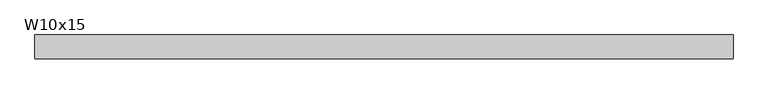
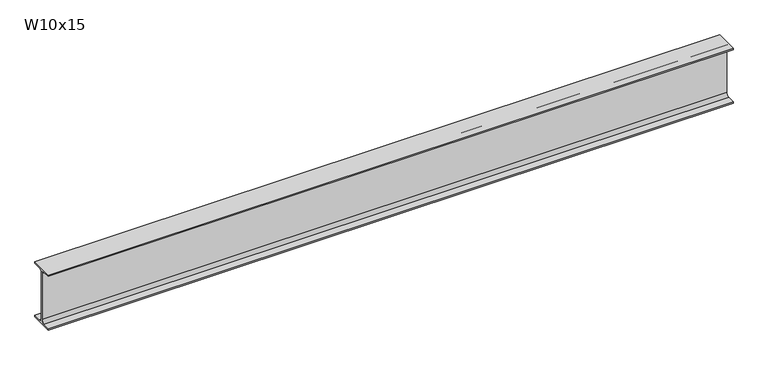
"""IFC4 building model written with IfcOpenShell, lengths in millimetres: beam geometry, RME W-Wide Flange : W10x15."""

from ifc_helpers import new_model, si_unit, point, frame, frame_2d, origin, place, context, project, spatial, polyline, circle_curve, trimmed, segment, composite_curve, outline, extrude, source, transform, mapped, element, save


def w10x15_925daf79(model_context):
    return source(origin(), model_context, "Body", "SweptSolid", [
        extrude(outline(composite_curve([segment(polyline([(50.8, -120.142), (50.8, -127.0), (-50.8, -127.0), (-50.8, -120.142), (-16.7005, -120.142)]), True, "CONTINUOUS"), segment(trimmed(circle_curve(frame_2d((-16.7005, -106.3625)), 13.7795), [point((-16.7005, -120.142))], [point((-2.921, -106.3625))], True, "CARTESIAN"), True, "CONTINUOUS"), segment(polyline([(-2.921, -106.3625), (-2.921, 106.3625)]), True, "CONTINUOUS"), segment(trimmed(circle_curve(frame_2d((-16.7005, 106.3625)), 13.7795), [point((-2.921, 106.3625))], [point((-16.7005, 120.142))], True, "CARTESIAN"), True, "CONTINUOUS"), segment(polyline([(-16.7005, 120.142), (-50.8, 120.142), (-50.8, 127.0), (50.8, 127.0), (50.8, 120.142), (16.7005, 120.142)]), True, "CONTINUOUS"), segment(trimmed(circle_curve(frame_2d((16.7005, 106.3625)), 13.7795), [point((16.7005, 120.142))], [point((2.921, 106.3625))], True, "CARTESIAN"), True, "CONTINUOUS"), segment(polyline([(2.921, 106.3625), (2.921, -106.3625)]), True, "CONTINUOUS"), segment(trimmed(circle_curve(frame_2d((16.7005, -106.3625)), 13.7795), [point((2.921, -106.3625))], [point((16.7005, -120.142))], True, "CARTESIAN"), True, "CONTINUOUS"), segment(polyline([(16.7005, -120.142), (50.8, -120.142)]), True, "CONTINUOUS")], self_intersect=False)), frame((-1518.6542329, 0.0, 0.0), z_axis=(1.0, 0.0, 0.0), x_axis=(0.0, 1.0, 0.0)), (0.0, 0.0, 1.0), 2991.0372286),
    ])


if __name__ == "__main__":
    model = new_model("IFC4")
    model_context = context("Model", 3, world=origin())
    ifc_project = project(units=[si_unit("LENGTHUNIT", "METRE", prefix="MILLI")], contexts=[model_context])
    site = spatial("IfcSite", under=ifc_project)
    building = spatial("IfcBuilding", under=site)
    placement = place(None, origin())
    w10x15_shape = w10x15_925daf79(model_context)
    element("IfcBeam", 1, ObjectType="RME W-Wide Flange : W10x15", at=placement, inside=building, context=model_context, shape_type="MappedRepresentation", body=[
        mapped(w10x15_shape, transform((0.0, 0.0, 0.0), x_axis=(1.0, 0.0, 0.0), y_axis=(0.0, 1.0, 0.0), z_axis=(0.0, 0.0, 1.0))),
    ])
    save(model, "model.ifc")

# Revit data of these elements
# Type "RME W-Wide Flange : W10x15"
#   WELD P [instance default] = ""
#   WELD LE [instance default] = ""
#   WELD D [instance default] = ""
#   TOP SECTION SIZE [instance default] = ""
#   TOP SECTION LENGTH [instance default] = ""
#   REMARKS [instance default] = ""
#   REINF TYPE [instance default] = ""
#   Nominal Size = "W24"
#   End Bearing Capacity [instance default] = ""
#   BOT SECTION SIZE [instance default] = ""
#   BOT SECTION LENGTH [instance default] = ""
#   Assembly Code = "B10"
#   W = 15
#   Start Extension Calculation [instance default] = 10' - 0"
#   Start Extension [instance default] = -0' - 0 1/2"
#   End Extension Calculation [instance default] = 10' - 0"
#   End Extension [instance default] = -0' - 0 1/2"
#   Length [instance default] = 5' - 0"
#   bf = 0' - 4"
#   d = 0' - 10"
#   k = 0' - 0 13/16"
#   k2 = 0' - 0.5425"
#   tf = 0' - 0.27"
#   tw = 0' - 0.23"
#   A = 0.030625 SF
#   Structural Material [instance default] = Metal - Steel - ASTM A992
# Element 1 (IfcBeam, "RME W-Wide Flange : W10x15")
#   Length = 9' - 6.00377"
#   Materials on its faces: "Metal - Steel - ASTM A992"
# Materials
#   "Metal - Steel - ASTM A992": class "Metal", colour RGB 255 128 0, transparency 0
